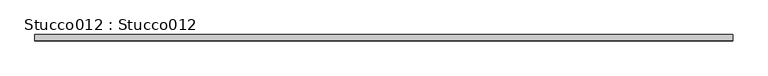
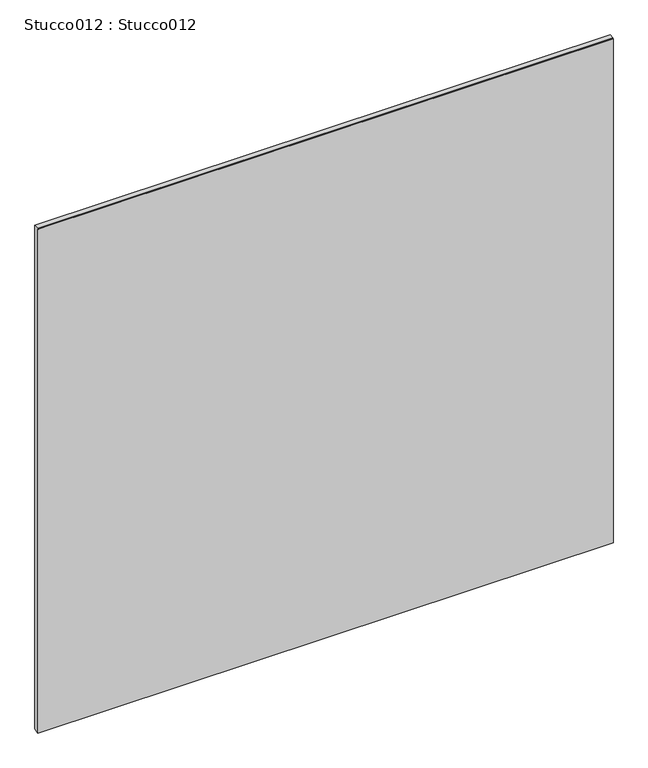
"""IFC4 building model written with IfcOpenShell, lengths in millimetres: proxy geometry, Stucco012 : Stucco012."""

from ifc_helpers import new_model, si_unit, frame, origin, place, context, project, spatial, polyline, outline, extrude, source, transform, mapped, element, save


def stucco012_stucco012_79def4a0(model_context):
    return source(origin(), model_context, "Body", "SweptSolid", [
        extrude(outline(polyline([(-4664.2116774, 36545.734375), (-4681.9917972, 36540.0208437), (-4681.9917972, 38391.9884812), (-4680.7217972, 38391.9884812), (-4680.7217972, 38395.4682812), (-4664.2116774, 38395.4682812), (-4664.2116774, 36545.734375)])), frame((12383.0178845, 0.0, 0.0), z_axis=(1.0, 0.0, 0.0), x_axis=(0.0, 1.0, 0.0)), (0.0, 0.0, 1.0), 2000.0),
    ])


if __name__ == "__main__":
    model = new_model("IFC4")
    model_context = context("Model", 3, world=origin())
    ifc_project = project(units=[si_unit("LENGTHUNIT", "METRE", prefix="MILLI")], contexts=[model_context])
    site = spatial("IfcSite", under=ifc_project)
    building = spatial("IfcBuilding", under=site)
    placement = place(None, origin())
    stucco012_stucco012_shape = stucco012_stucco012_79def4a0(model_context)
    element("IfcBuildingElementProxy", 1, Name="Stucco012 : Stucco012", ObjectType="Stucco012 : Stucco012", at=placement, inside=building, context=model_context, shape_type="MappedRepresentation", body=[
        mapped(stucco012_stucco012_shape, transform((0.0, 0.0, 0.0), x_axis=(1.0, 0.0, 0.0), y_axis=(0.0, 1.0, 0.0), z_axis=(0.0, 0.0, 1.0))),
    ])
    save(model, "model.ifc")

# Revit data of these elements
# Type "Stucco012 : Stucco012"
#   NameOverride = "Stucco012"
# Element 1 (IfcBuildingElementProxy, "Stucco012 : Stucco012")
#   Materials on its faces: "7/8\" SMOOTH TROWEL EXTERIOR STUCCO"
# Materials
#   "7/8\" SMOOTH TROWEL EXTERIOR STUCCO": class "Unassigned", colour RGB 255 255 255, transparency 0, Cost = 0
